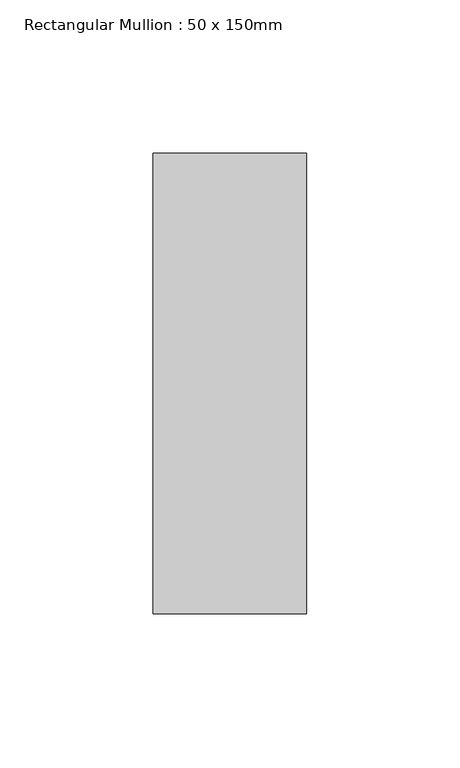
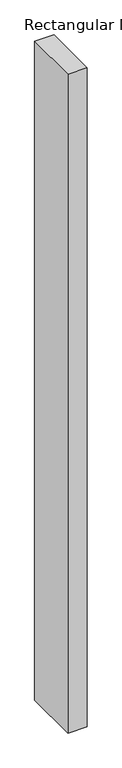
"""IFC4 building model written with IfcOpenShell, lengths in millimetres: member geometry, Rectangular Mullion : 50 x 150mm."""

from ifc_helpers import new_model, si_unit, frame, origin, place, context, project, spatial, polyline, outline, extrude, source, transform, mapped, element, save


def rectangular_mullion_50_x_150mm_84b4b286(model_context):
    return source(origin(), model_context, "Body", "SweptSolid", [
        extrude(outline(polyline([(0.0, 75.0), (0.0, -75.0), (-50.0, -75.0), (-50.0, 75.0), (0.0, 75.0)])), frame((0.0, 0.0, -1813.8888891), z_axis=(0.0, 0.0, 1.0), x_axis=(1.0, 0.0, 0.0)), (0.0, 0.0, 1.0), 1813.8888891),
    ])


if __name__ == "__main__":
    model = new_model("IFC4")
    model_context = context("Model", 3, world=origin())
    ifc_project = project(units=[si_unit("LENGTHUNIT", "METRE", prefix="MILLI")], contexts=[model_context])
    site = spatial("IfcSite", under=ifc_project)
    building = spatial("IfcBuilding", under=site)
    placement = place(None, origin())
    rectangular_mullion_50_x_150mm_shape = rectangular_mullion_50_x_150mm_84b4b286(model_context)
    element("IfcMember", 1, ObjectType="Rectangular Mullion : 50 x 150mm", at=placement, inside=building, context=model_context, shape_type="MappedRepresentation", body=[
        mapped(rectangular_mullion_50_x_150mm_shape, transform((0.0, 0.0, 0.0), x_axis=(1.0, 0.0, 0.0), y_axis=(0.0, 1.0, 0.0), z_axis=(0.0, 0.0, 1.0))),
    ])
    save(model, "model.ifc")

# Revit data of these elements
# Type "Rectangular Mullion : 50 x 150mm"
#   built-in parameter 1007304 = 0.492126 (stored number, unit not read)
#   built-in parameter 1007301 = 0.082021 (stored number, unit not read)
#   built-in parameter 1007300 = 0.082021 (stored number, unit not read)
# Element 1 (IfcMember, "Rectangular Mullion : 50 x 150mm")
#   Materials on its faces: "Metal - Aluminium"
# Materials
#   "Metal - Aluminium": class "Metal", colour RGB 247 247 247, transparency 0
